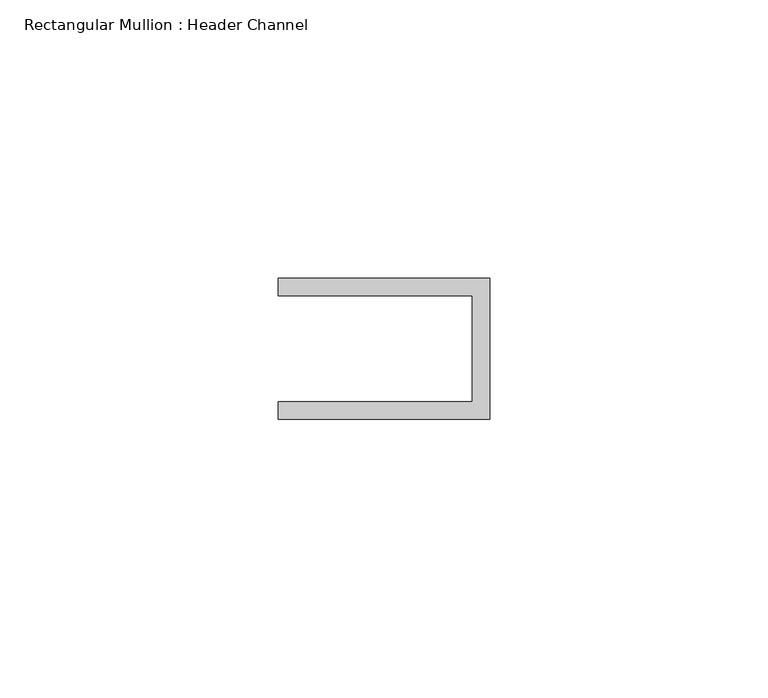
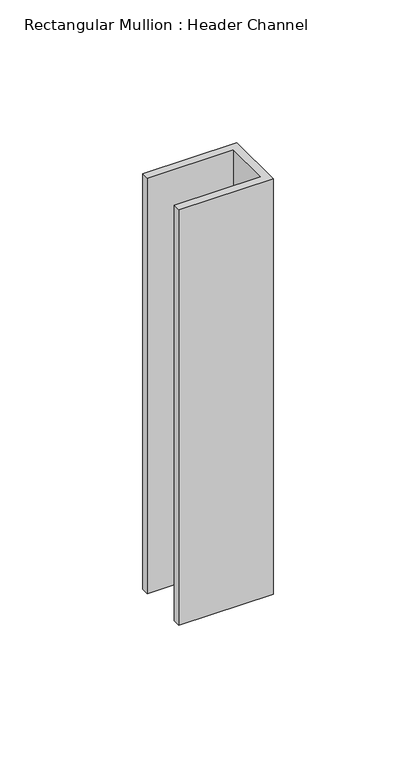
"""IFC4 building model written with IfcOpenShell, lengths in millimetres: member geometry, Rectangular Mullion : Header Channel."""

from ifc_helpers import new_model, si_unit, frame, origin, place, context, project, spatial, polyline, outline, extrude, source, transform, mapped, element, save


def rectangular_mullion_header_channel_e907cd1b(model_context):
    return source(origin(), model_context, "Body", "SweptSolid", [
        extrude(outline(polyline([(0.0, -12.7), (-38.1, -12.7), (-38.1, -9.525), (-3.175, -9.525), (-3.175, 9.525), (-38.1, 9.525), (-38.1, 12.7), (0.0, 12.7), (0.0, -12.7)])), frame((0.0, 0.0, -177.8), z_axis=(0.0, 0.0, 1.0), x_axis=(1.0, 0.0, 0.0)), (0.0, 0.0, 1.0), 177.8),
    ])


if __name__ == "__main__":
    model = new_model("IFC4")
    model_context = context("Model", 3, world=origin())
    ifc_project = project(units=[si_unit("LENGTHUNIT", "METRE", prefix="MILLI")], contexts=[model_context])
    site = spatial("IfcSite", under=ifc_project)
    building = spatial("IfcBuilding", under=site)
    placement = place(None, origin())
    rectangular_mullion_header_channel_shape = rectangular_mullion_header_channel_e907cd1b(model_context)
    element("IfcMember", 1, ObjectType="Rectangular Mullion : Header Channel", at=placement, inside=building, context=model_context, shape_type="MappedRepresentation", body=[
        mapped(rectangular_mullion_header_channel_shape, transform((0.0, 0.0, 0.0), x_axis=(1.0, 0.0, 0.0), y_axis=(0.0, 1.0, 0.0), z_axis=(0.0, 0.0, 1.0))),
    ])
    save(model, "model.ifc")

# Revit data of these elements
# Type "Rectangular Mullion : Header Channel"
#   built-in parameter 1007322 = 0.0833333 (stored number, unit not read)
#   built-in parameter 1007321 = -0.03125 (stored number, unit not read)
#   built-in parameter 1007320 = 0.0416667 (stored number, unit not read)
# Element 1 (IfcMember, "Rectangular Mullion : Header Channel")
#   Materials on its faces: "ALUM"
# Materials
#   "ALUM": class "Generic", colour RGB 157 157 157, transparency 0, Cost = 0
